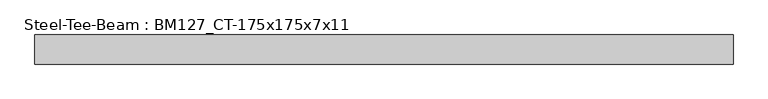
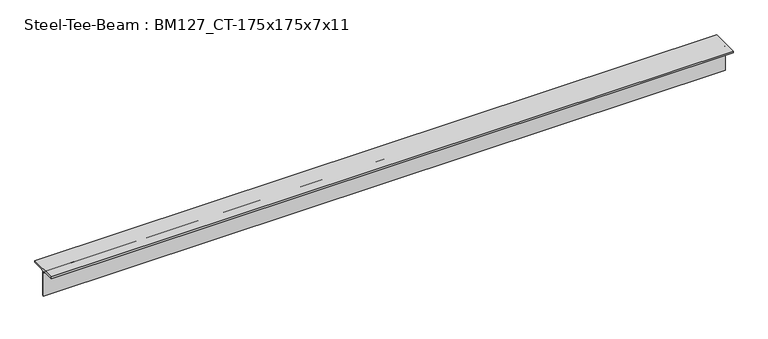
"""IFC4 building model written with IfcOpenShell, lengths in millimetres: beam geometry, Steel-Tee-Beam : BM127_CT-175x175x7x11."""

import ifcopenshell
import ifcopenshell.guid

model = None  # the IFC model being written
_history = None  # IfcOwnerHistory: only IFC2X3 demands one
_inside = {}  # id of a spatial element -> (the spatial element, [elements in it])
_under = {}  # id of a project, library or spatial element -> (it, [spatial elements below it])
_declared = {}  # id of a project -> (the project, [libraries it declares])
_typed = {}  # id of a type object -> (the type object, [elements of that type])
_made_of = {}  # id of a material, layer set ... -> (it, [elements and type objects made of it])


def new_model(schema):
    """Start an empty IFC model of exactly this schema.

    Asked for "IFC4X3", IfcOpenShell would pick the latest addendum, in which some entities
    have other attributes; the version numbers below select the first issue.
    IFC2X3 requires an IfcOwnerHistory on every rooted entity: one is made here for all.
    """
    global model, _history
    if schema == "IFC4X3":
        model = ifcopenshell.file(schema_version=(4, 3, 0, 0))
    else:
        model = ifcopenshell.file(schema=schema)
    _inside.clear()
    _under.clear()
    _declared.clear()
    _typed.clear()
    _made_of.clear()
    _history = None
    if model.schema == "IFC2X3":
        org = make("IfcOrganization", Name="unknown")
        user = make(
            "IfcPersonAndOrganization",
            ThePerson=make("IfcPerson", FamilyName="unknown"),
            TheOrganization=org,
        )
        app = make(
            "IfcApplication",
            ApplicationDeveloper=org,
            Version="unknown",
            ApplicationFullName="unknown",
            ApplicationIdentifier="unknown",
        )
        _history = make(
            "IfcOwnerHistory",
            OwningUser=user,
            OwningApplication=app,
            ChangeAction="ADDED",
            CreationDate=0,
        )
    return model


def make(cls, **values):
    """One entity of the class cls with the attributes given. An attribute that is None is left unset."""
    return model.create_entity(
        cls, **{name: value for name, value in values.items() if value is not None}
    )


def rooted(cls, **values):
    """An entity with a GlobalId (a new one), such as an element, a storey or a relation."""
    return make(cls, GlobalId=ifcopenshell.guid.new(), OwnerHistory=_history, **values)


def si_unit(unit_type, name, prefix=None):
    """IfcSIUnit, for example si_unit("LENGTHUNIT", "METRE", prefix="MILLI")."""
    return make("IfcSIUnit", UnitType=unit_type, Prefix=prefix, Name=name)


def assignment(units):
    """IfcUnitAssignment: the units of a project."""
    return None if units is None else make("IfcUnitAssignment", Units=units)


def point(xyz):
    """IfcCartesianPoint."""
    return None if xyz is None else make("IfcCartesianPoint", Coordinates=xyz)


def direction(xyz):
    """IfcDirection."""
    return None if xyz is None else make("IfcDirection", DirectionRatios=xyz)


def frame(location, z_axis=None, x_axis=None):
    """IfcAxis2Placement3D, a coordinate frame: its origin and axes. An axis left out is left unset."""
    return make(
        "IfcAxis2Placement3D",
        Location=point(location),
        Axis=direction(z_axis),
        RefDirection=direction(x_axis),
    )


def frame_2d(location, x_axis=None):
    """IfcAxis2Placement2D, a coordinate frame in the plane: its origin and x axis."""
    return make(
        "IfcAxis2Placement2D", Location=point(location), RefDirection=direction(x_axis)
    )


def origin():
    """The frame at (0, 0, 0) with its axes left unset."""
    return frame((0.0, 0.0, 0.0))


def place(relative_to, where):
    """IfcLocalPlacement: puts the frame where relative to a parent placement (None: the world)."""
    return make(
        "IfcLocalPlacement", PlacementRelTo=relative_to, RelativePlacement=where
    )


def context(
    kind, dimensions, precision=None, world=None, true_north=None, identifier=None
):
    """IfcGeometricRepresentationContext, for example the 3D "Model" context."""
    return make(
        "IfcGeometricRepresentationContext",
        ContextIdentifier=identifier,
        ContextType=kind,
        CoordinateSpaceDimension=dimensions,
        Precision=precision,
        WorldCoordinateSystem=world,
        TrueNorth=true_north,
    )


def project(units=None, contexts=None):
    """IfcProject with its units and contexts."""
    return rooted(
        "IfcProject",
        Name="project",
        RepresentationContexts=contexts,
        UnitsInContext=assignment(units),
    )


def spatial(cls, under=None, at=None, **own):
    """A site, building, storey or space (cls), placed at a placement, below another one or the project."""
    s = rooted(cls, ObjectPlacement=at, **own)
    if under is not None:
        _under.setdefault(under.id(), (under, []))[1].append(s)
    return s


def polyline(points):
    """IfcPolyline through the points."""
    return make("IfcPolyline", Points=[point(p) for p in points])


def circle_curve(where, radius):
    """IfcCircle in the frame where."""
    return make("IfcCircle", Position=where, Radius=radius)


def trimmed(basis, trim1, trim2, sense, master):
    """IfcTrimmedCurve: the piece of a basis curve between two trims."""
    return make(
        "IfcTrimmedCurve",
        BasisCurve=basis,
        Trim1=trim1,
        Trim2=trim2,
        SenseAgreement=sense,
        MasterRepresentation=master,
    )


def segment(curve, same_sense, transition):
    """IfcCompositeCurveSegment."""
    return make(
        "IfcCompositeCurveSegment",
        Transition=transition,
        SameSense=same_sense,
        ParentCurve=curve,
    )


def composite_curve(segments, self_intersect=None):
    """IfcCompositeCurve: segments joined end to end."""
    return make("IfcCompositeCurve", Segments=segments, SelfIntersect=self_intersect)


def outline(outer, holes=None, kind="AREA"):
    """IfcArbitraryClosedProfileDef: a profile drawn as a closed curve; with holes, ...WithVoids."""
    if holes is None:
        return make("IfcArbitraryClosedProfileDef", ProfileType=kind, OuterCurve=outer)
    return make(
        "IfcArbitraryProfileDefWithVoids",
        ProfileType=kind,
        OuterCurve=outer,
        InnerCurves=holes,
    )


def extrude(swept, where, along, depth):
    """IfcExtrudedAreaSolid: the profile swept, set in the frame where, extruded along a direction by depth."""
    return make(
        "IfcExtrudedAreaSolid",
        SweptArea=swept,
        Position=where,
        ExtrudedDirection=direction(along),
        Depth=depth,
    )


def shape(context_of_items, identifier, shape_type, items):
    """IfcShapeRepresentation: the items that make up one representation, for example the "Body"."""
    return make(
        "IfcShapeRepresentation",
        ContextOfItems=context_of_items,
        RepresentationIdentifier=identifier,
        RepresentationType=shape_type,
        Items=items,
    )


def source(mapping_origin, context_of_items, identifier, shape_type, items):
    """IfcRepresentationMap: a shape defined once, which mapped items show again and again."""
    return make(
        "IfcRepresentationMap",
        MappingOrigin=mapping_origin,
        MappedRepresentation=shape(context_of_items, identifier, shape_type, items),
    )


def transform(
    local_origin,
    x_axis=None,
    y_axis=None,
    z_axis=None,
    scale=None,
    scale2=None,
    scale3=None,
    uniform=True,
):
    """IfcCartesianTransformationOperator3D, or its non-uniform kind. x_axis, y_axis, z_axis: its Axis1, 2, 3."""
    if uniform:
        return make(
            "IfcCartesianTransformationOperator3D",
            Axis1=direction(x_axis),
            Axis2=direction(y_axis),
            LocalOrigin=point(local_origin),
            Scale=scale,
            Axis3=direction(z_axis),
        )
    return make(
        "IfcCartesianTransformationOperator3DnonUniform",
        Axis1=direction(x_axis),
        Axis2=direction(y_axis),
        LocalOrigin=point(local_origin),
        Scale=scale,
        Axis3=direction(z_axis),
        Scale2=scale2,
        Scale3=scale3,
    )


def mapped(mapping_source, mapping_target):
    """IfcMappedItem: shows the shape of a source again, moved by a transform."""
    return make(
        "IfcMappedItem", MappingSource=mapping_source, MappingTarget=mapping_target
    )


def made_of(thing, what):
    """Note that an element or type object is made of a material, layer set ...; save() writes the relation."""
    if what is not None:
        _made_of.setdefault(what.id(), (what, []))[1].append(thing)
    return thing


def element(
    cls,
    number,
    at=None,
    inside=None,
    cuts=None,
    type_object=None,
    material=None,
    context=None,
    identifier="Body",
    shape_type=None,
    held_by="IfcProductDefinitionShape",
    body=None,
    shapes=None,
    **own,
):
    """One element of the class cls, such as IfcWall. Its Tag is "e" and its number.

    at: its placement. inside: the storey or other place that contains it. cuts: it is an
    opening in that element (IfcRelVoidsElement). A single representation is given by context,
    identifier, shape_type and body (its items); several are given by shapes. held_by: the class
    of the entity that holds the representations. save() writes the other relations.
    """
    e = rooted(cls, Tag="e%d" % number, ObjectPlacement=at, **own)
    if body is not None:
        shapes = [shape(context, identifier, shape_type, body)]
    if shapes is not None:
        e.Representation = make(held_by, Representations=shapes)
    if inside is not None:
        _inside.setdefault(inside.id(), (inside, []))[1].append(e)
    if cuts is not None:
        rooted(
            "IfcRelVoidsElement", RelatingBuildingElement=cuts, RelatedOpeningElement=e
        )
    if type_object is not None:
        _typed.setdefault(type_object.id(), (type_object, []))[1].append(e)
    return made_of(e, material)


def aggregate(whole, parts):
    """IfcRelAggregates: a whole, such as a stair, and the parts it consists of."""
    return rooted("IfcRelAggregates", RelatingObject=whole, RelatedObjects=parts)


def save(model, path):
    """Write the relations noted so far, then the file.

    IfcRelAggregates (storeys below a building ...), IfcRelContainedInSpatialStructure (elements
    in a storey), IfcRelDefinesByType, IfcRelAssociatesMaterial and IfcRelDeclares: one each for
    every whole, place, type object, material and project.
    """
    for whole, parts in _under.values():
        aggregate(whole, parts)
    for where, things in _inside.values():
        rooted(
            "IfcRelContainedInSpatialStructure",
            RelatedElements=things,
            RelatingStructure=where,
        )
    for kind, things in _typed.values():
        rooted("IfcRelDefinesByType", RelatedObjects=things, RelatingType=kind)
    for what, things in _made_of.values():
        rooted("IfcRelAssociatesMaterial", RelatedObjects=things, RelatingMaterial=what)
    for by, libraries in _declared.values():
        rooted("IfcRelDeclares", RelatingContext=by, RelatedDefinitions=libraries)
    model.write(path)


def steel_tee_beam_bm127_ct_175x175x7x11_e8e1f4b2(model_context):
    return source(origin(), model_context, "Body", "SweptSolid", [
        extrude(outline(composite_curve([segment(polyline([(-87.5, 87.5), (87.5, 87.5), (87.5, 76.5), (17.5, 76.5)]), True, "CONTINUOUS"), segment(trimmed(circle_curve(frame_2d((17.5, 62.5)), 14.0), [point((17.5, 76.5))], [point((3.5, 62.5))], True, "CARTESIAN"), True, "CONTINUOUS"), segment(polyline([(3.5, 62.5), (3.5, -87.5), (-3.5, -87.5), (-3.5, 62.5)]), True, "CONTINUOUS"), segment(trimmed(circle_curve(frame_2d((-17.5, 62.5)), 14.0), [point((-3.5, 62.5))], [point((-17.5, 76.5))], True, "CARTESIAN"), True, "CONTINUOUS"), segment(polyline([(-17.5, 76.5), (-87.5, 76.5), (-87.5, 87.5)]), True, "CONTINUOUS")], self_intersect=False)), frame((-1998.4928423, 0.0, 0.0), z_axis=(1.0, 0.0, 0.0), x_axis=(0.0, 1.0, 0.0)), (0.0, 0.0, 1.0), 4194.118334),
    ])


if __name__ == "__main__":
    model = new_model("IFC4")
    model_context = context("Model", 3, world=origin())
    ifc_project = project(units=[si_unit("LENGTHUNIT", "METRE", prefix="MILLI")], contexts=[model_context])
    site = spatial("IfcSite", under=ifc_project)
    building = spatial("IfcBuilding", under=site)
    placement = place(None, origin())
    steel_tee_beam_bm127_ct_175x175x7x11_shape = steel_tee_beam_bm127_ct_175x175x7x11_e8e1f4b2(model_context)
    element("IfcBeam", 1, ObjectType="Steel-Tee-Beam : BM127_CT-175x175x7x11", at=placement, inside=building, context=model_context, shape_type="MappedRepresentation", body=[
        mapped(steel_tee_beam_bm127_ct_175x175x7x11_shape, transform((0.0, 0.0, 0.0), x_axis=(1.0, 0.0, 0.0), y_axis=(0.0, 1.0, 0.0), z_axis=(0.0, 0.0, 1.0))),
    ])
    save(model, "model.ifc")

# Revit data of these elements
# Type "Steel-Tee-Beam : BM127_CT-175x175x7x11"
#   Surface Area = 0.00 m²/m
#   Section Area = 31.57 cm²
#   Mass per Unit Length = 24.80 kg/m
#   Length [instance default] = 1524 mm
#   bf = 175 mm
#   d = 175 mm
#   k = 25 mm
#   kr = 14 mm
#   tf = 11 mm
#   tw = 7 mm
#   hec_material4 [instance default] = none
#   hec_material3 [instance default] = none
#   hec_material2 [instance default] = none
#   hec_material1 [instance default] = none
#   Structural Material [instance default] = Steel, 45-345
#   Assembly Code = ""
# Element 1 (IfcBeam, "Steel-Tee-Beam : BM127_CT-175x175x7x11")
#   hec_material3 = F01AC000-00002_Building/Shelter Fire Proofing Work_Intumescent Coating Type_1 hr. rating (UL 1709))
#   hec_material2 = S01AA010-00002_Main Steel Structure Fabrication Work_Shelter/Building_Steel Painting/Coating_for Fireproofed Steel Surface, Surface Preparation & Primer Coat
#   hec_material1 = S03AA029-00001_Main Steel Structure Erection Work_Shelter/Building_Light Steel
#   Structural Material = S01AA003-00001_Main Steel Structure Fabrication Work_Shelter/Building_Light Steel - Standard
#   Materials on its faces: "S01AA003-00001_Main Steel Structure Fabrication Work_Shelter/Building_Light Steel - Standard"
# Materials
#   "Steel, 45-345": class "Metal", colour RGB 189 187 185, transparency 0, Description = "Steel 345 MPa", Cost = 0
#   "S01AA003-00001_Main Steel Structure Fabrication Work_Shelter/Building_Light Steel - Standard": class "Metal", colour RGB 120 120 120, transparency 0, Comments = "(30KG/M>Weight)", Description = "Structural steel 50ksi", W00) Work Master Code = "S01AA003-00001", W01) Work Master_Lv1 = "Main Steel Structure Fabrication Work", W02) Work Master_Lv2 = "Shelter/Building", W03) Work Master_Spec.1 = "Light Steel - Standard (30KG/M>Weight)", Cost = 0
#   "F01AC000-00002_Building/Shelter Fire Proofing Work_Intumescent Coating Type_1 hr. rating (UL 1709))": class "Metal", colour RGB 255 128 128, transparency 0, Description = "Paint finished steel", W00) Work Master Code = "F01AC000-00002", W01) Work Master_Lv1 = "Building/Shelter Fire Proofing Work", W02) Work Master_Lv2 = "Intumescent Coating Type", W03) Work Master_Spec.1 = "1 hr. rating (UL 1709)", Cost = 0
#   "S01AA010-00002_Main Steel Structure Fabrication Work_Shelter/Building_Steel Painting/Coating_for Fireproofed Steel Surface, Surface Preparation & Primer Coat": class "Metal", colour RGB 120 120 120, transparency 0, Description = "Paint finished steel", W00) Work Master Code = "SS01AA010-00002", W01) Work Master_Lv1 = "Main Steel Structure Fabrication Work", W02) Work Master_Lv2 = "Shelter/Building", W03) Work Master_Spec.1 = "Steel Painting/Coating", W04) Work Master_Spec.2 = "for Fireproofed Steel Surface, Surface Preparation & Primer Coat", Cost = 0
#   "S03AA029-00001_Main Steel Structure Erection Work_Shelter/Building_Light Steel": class "Metal", colour RGB 120 120 120, transparency 0, Comments = "(30KG/M>Weight)", Description = "Structural steel 50ksi", W00) Work Master Code = "S03AA029-00001", W01) Work Master_Lv1 = "Main Steel Structure Erection Work", W02) Work Master_Lv2 = "Shelter/Building", W03) Work Master_Spec.1 = "Light Steel (30KG/M>Weight)", Cost = 0
